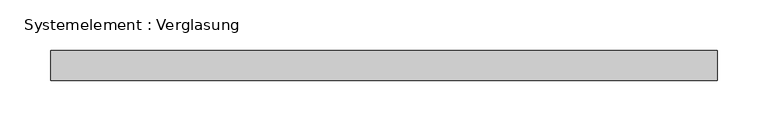
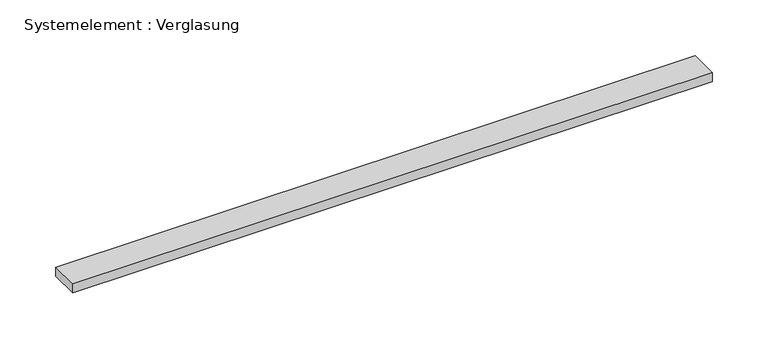
"""IFC4 building model written with IfcOpenShell, lengths in millimetres: plate geometry, Systemelement : Verglasung."""

from ifc_helpers import new_model, si_unit, origin, origin_with_axes, place, context, project, spatial, polyline, outline, extrude, source, transform, mapped, element, save


def systemelement_verglasung_0eadd769(model_context):
    return source(origin(), model_context, "Body", "SweptSolid", [
        extrude(outline(polyline([(330.143661, -15.0), (-330.143661, -15.0), (-330.143661, 15.0), (330.143661, 15.0), (330.143661, -15.0)])), origin_with_axes(), (0.0, 0.0, 1.0), 10.0),
    ])


if __name__ == "__main__":
    model = new_model("IFC4")
    model_context = context("Model", 3, world=origin())
    ifc_project = project(units=[si_unit("LENGTHUNIT", "METRE", prefix="MILLI")], contexts=[model_context])
    site = spatial("IfcSite", under=ifc_project)
    building = spatial("IfcBuilding", under=site)
    placement = place(None, origin())
    systemelement_verglasung_shape = systemelement_verglasung_0eadd769(model_context)
    element("IfcPlate", 1, ObjectType="Systemelement : Verglasung", at=placement, inside=building, context=model_context, shape_type="MappedRepresentation", body=[
        mapped(systemelement_verglasung_shape, transform((0.0, 0.0, 0.0), x_axis=(1.0, 0.0, 0.0), y_axis=(0.0, 1.0, 0.0), z_axis=(0.0, 0.0, 1.0))),
    ])
    save(model, "model.ifc")

# Revit data of these elements
# Type "Systemelement : Verglasung"
#   Construction Type Id = "GSP4R"
#   Analytic Construction = "1/8 Zoll Pilkington-Verglasung einfach"
#   Visual Light Transmittance = 0.9
#   Solar Heat Gain Coefficient = 0.86
#   Heat Transfer Coefficient (U) = 6.7069 W/(m²·K)
# Element 1 (IfcPlate, "Systemelement : Verglasung")
#   Materials on its faces: "Glas"
# Materials
#   "Glas": class "Glas", colour RGB 0 0 255, transparency 0.75, Comments = "Render-Darstellung nicht aktualisiert ", Cost = 0
